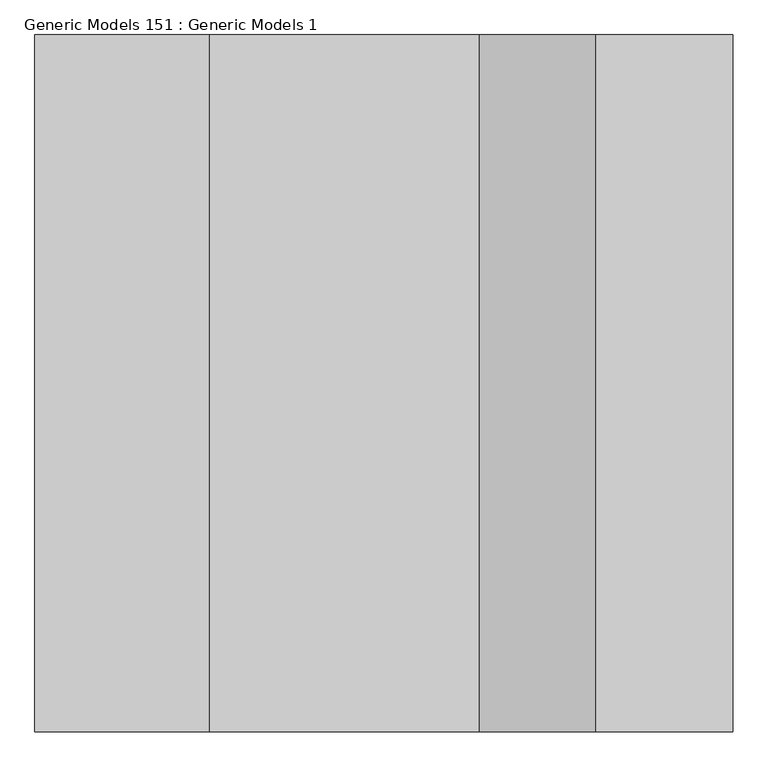
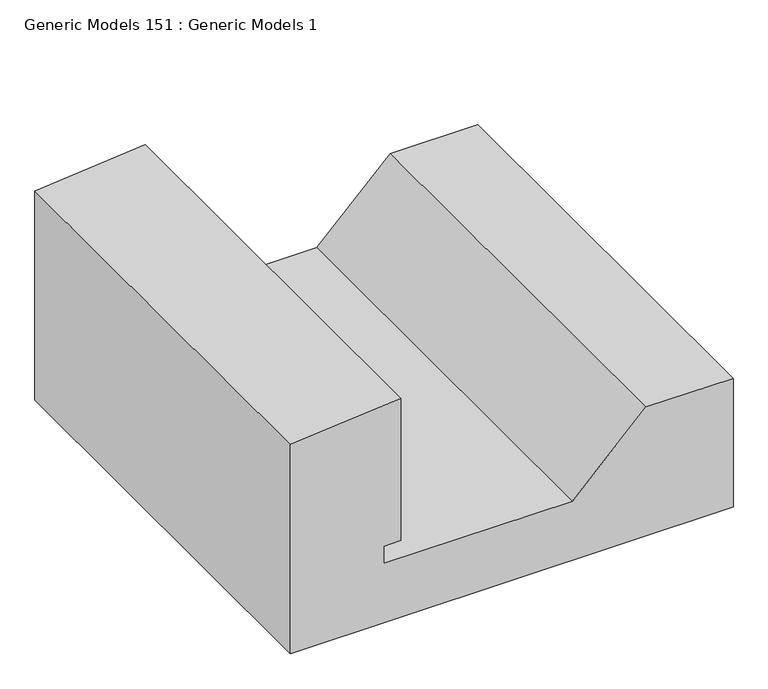
"""IFC4 building model written with IfcOpenShell, lengths in millimetres: proxy geometry, Generic Models 151 : Generic Models 1."""

from ifc_helpers import new_model, si_unit, frame, origin, place, context, project, spatial, polyline, outline, extrude, source, transform, mapped, element, save


def generic_models_151_generic_models_1_08f1ca75(model_context):
    return source(origin(), model_context, "Body", "SweptSolid", [
        extrude(outline(polyline([(-76.2, 51566.7625), (-685.8, 51566.7625), (-685.8, 52787.3395874), (-310.1710164, 52787.3395874), (-310.1710164, 52546.8563593), (-513.3710164, 52343.6563593), (-513.3710164, 51824.8420742), (-462.5710164, 51824.8420742), (-462.5710164, 51871.5625), (-47.9216734, 51871.5625), (-76.2, 51566.7625)])), frame((0.0, 0.0, 0.0), z_axis=(0.0, 1.0, 0.0), x_axis=(0.0, 0.0, 1.0)), (0.0, 0.0, 1.0), 1219.2),
    ])


if __name__ == "__main__":
    model = new_model("IFC4")
    model_context = context("Model", 3, world=origin())
    ifc_project = project(units=[si_unit("LENGTHUNIT", "METRE", prefix="MILLI")], contexts=[model_context])
    site = spatial("IfcSite", under=ifc_project)
    building = spatial("IfcBuilding", under=site)
    placement = place(None, origin())
    generic_models_151_generic_models_1_shape = generic_models_151_generic_models_1_08f1ca75(model_context)
    element("IfcBuildingElementProxy", 1, Name="Generic Models 151 : Generic Models 1", ObjectType="Generic Models 151 : Generic Models 1", at=placement, inside=building, context=model_context, shape_type="MappedRepresentation", body=[
        mapped(generic_models_151_generic_models_1_shape, transform((0.0, 0.0, 0.0), x_axis=(1.0, 0.0, 0.0), y_axis=(0.0, 1.0, 0.0), z_axis=(0.0, 0.0, 1.0))),
    ])
    save(model, "model.ifc")

# Revit data of these elements
# Element 1 (IfcBuildingElementProxy, "Generic Models 151 : Generic Models 1")
#   Materials on its faces: "GRADE (SLOPE 2% MIN AWAY FROM BUILDING)"
# Materials
#   "GRADE (SLOPE 2% MIN AWAY FROM BUILDING)": class "Generic", colour RGB 156 184 169, transparency 0, Description = "Soil", Cost = 0
